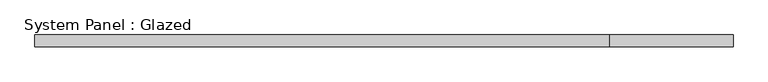
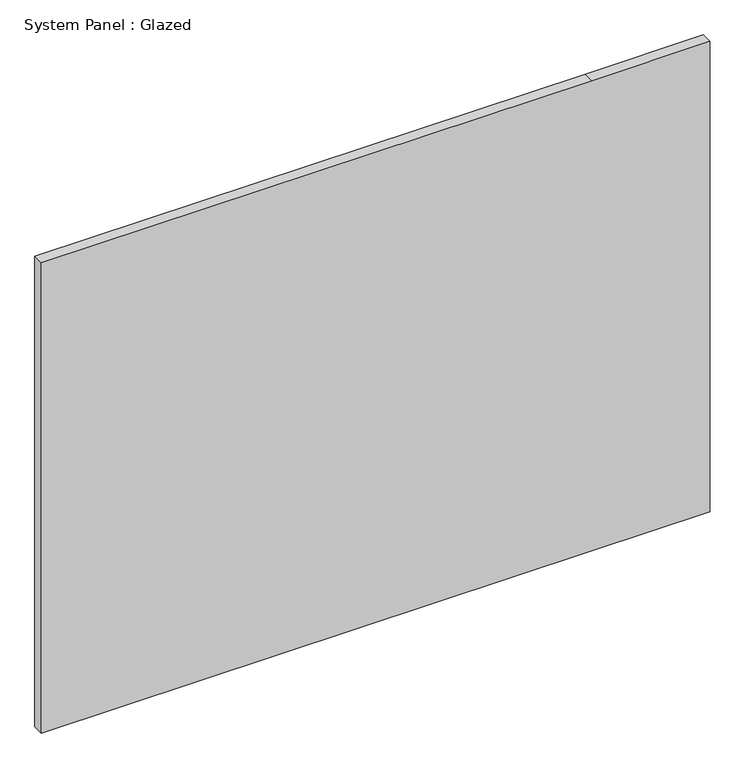
"""IFC4 building model written with IfcOpenShell, lengths in millimetres: plate geometry, System Panel : Glazed."""

from ifc_helpers import new_model, si_unit, frame, origin, place, context, project, spatial, polyline, outline, extrude, source, transform, mapped, element, save


def system_panel_glazed_fabe228a(model_context):
    return source(origin(), model_context, "Body", "SweptSolid", [
        extrude(outline(polyline([(0.0, -756.44375), (0.0, 488.95), (0.0, 756.44375), (1123.95, 756.44375), (1123.95, 488.95), (1123.95, -756.44375), (0.0, -756.44375)])), frame((0.0, -44.45, 0.0), z_axis=(0.0, 1.0, 0.0), x_axis=(0.0, 0.0, 1.0)), (0.0, 0.0, 1.0), 25.4),
    ])


if __name__ == "__main__":
    model = new_model("IFC4")
    model_context = context("Model", 3, world=origin())
    ifc_project = project(units=[si_unit("LENGTHUNIT", "METRE", prefix="MILLI")], contexts=[model_context])
    site = spatial("IfcSite", under=ifc_project)
    building = spatial("IfcBuilding", under=site)
    placement = place(None, origin())
    system_panel_glazed_shape = system_panel_glazed_fabe228a(model_context)
    element("IfcPlate", 1, ObjectType="System Panel : Glazed", at=placement, inside=building, context=model_context, shape_type="MappedRepresentation", body=[
        mapped(system_panel_glazed_shape, transform((0.0, 0.0, 0.0), x_axis=(1.0, 0.0, 0.0), y_axis=(0.0, 1.0, 0.0), z_axis=(0.0, 0.0, 1.0))),
    ])
    save(model, "model.ifc")

# Revit data of these elements
# Element 1 (IfcPlate, "System Panel : Glazed")
#   Materials on its faces: "Glass"
# Materials
#   "Glass": class "Glass", colour RGB 0 128 192, transparency 0.75
